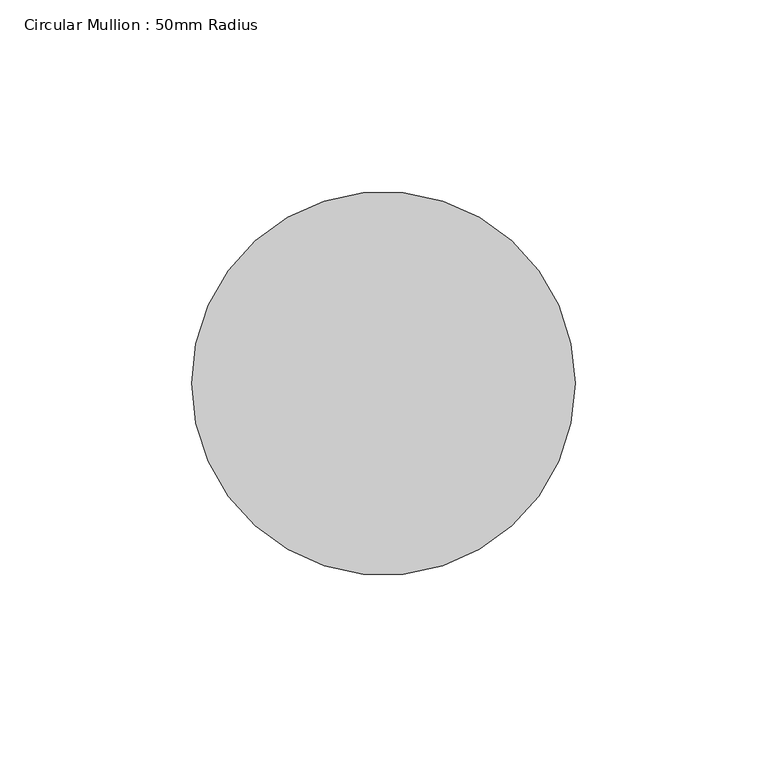
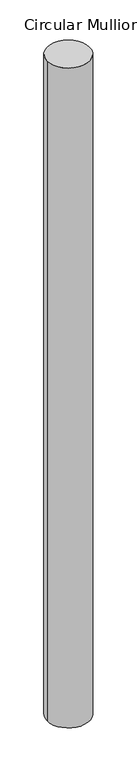
"""IFC4 building model written with IfcOpenShell, lengths in millimetres: member geometry, Circular Mullion : 50mm Radius."""

from ifc_helpers import new_model, si_unit, point, frame, origin, origin_2d, place, context, project, spatial, circle_curve, trimmed, segment, composite_curve, outline, extrude, source, transform, mapped, element, save


def circular_mullion_50mm_radius_96c2828a(model_context):
    return source(origin(), model_context, "Body", "SweptSolid", [
        extrude(outline(composite_curve([segment(trimmed(circle_curve(origin_2d(), 50.0), [point((50.0, 0.0))], [point((-50.0, 0.0))], False, "CARTESIAN"), True, "CONTINUOUS"), segment(trimmed(circle_curve(origin_2d(), 50.0), [point((-50.0, 0.0))], [point((50.0, 0.0))], False, "CARTESIAN"), True, "CONTINUOUS")], self_intersect=False)), frame((0.0, 0.0, -1646.8564236), z_axis=(0.0, 0.0, 1.0), x_axis=(1.0, 0.0, 0.0)), (0.0, 0.0, 1.0), 1646.8564236),
    ])


if __name__ == "__main__":
    model = new_model("IFC4")
    model_context = context("Model", 3, world=origin())
    ifc_project = project(units=[si_unit("LENGTHUNIT", "METRE", prefix="MILLI")], contexts=[model_context])
    site = spatial("IfcSite", under=ifc_project)
    building = spatial("IfcBuilding", under=site)
    placement = place(None, origin())
    circular_mullion_50mm_radius_shape = circular_mullion_50mm_radius_96c2828a(model_context)
    element("IfcMember", 1, ObjectType="Circular Mullion : 50mm Radius", at=placement, inside=building, context=model_context, shape_type="MappedRepresentation", body=[
        mapped(circular_mullion_50mm_radius_shape, transform((0.0, 0.0, 0.0), x_axis=(1.0, 0.0, 0.0), y_axis=(0.0, 1.0, 0.0), z_axis=(0.0, 0.0, 1.0))),
    ])
    save(model, "model.ifc")

# Revit data of these elements
# Type "Circular Mullion : 50mm Radius"
#   built-in parameter 1007350 = 0.164042 (stored number, unit not read)
# Element 1 (IfcMember, "Circular Mullion : 50mm Radius")
#   Materials on its faces: "Aluminium"
# Materials
#   "Aluminium": class "Metal", colour RGB 247 247 247, transparency 0, Description = "Aluminium 6061", Cost = 0
